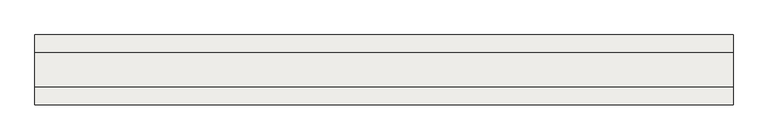
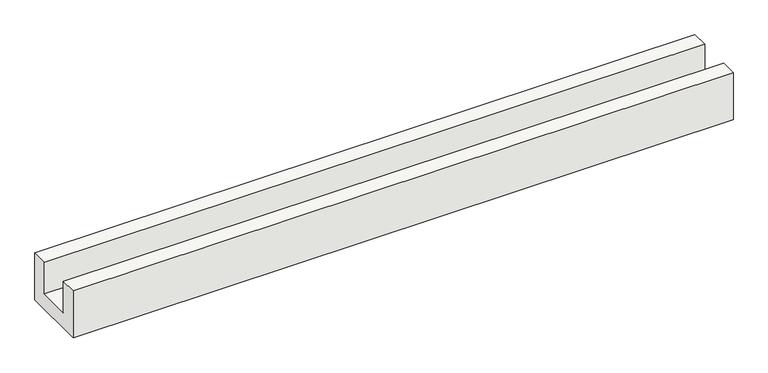
"""IFC4 building model written with IfcOpenShell, lengths in millimetres: slab geometry, 구조 기초 2 : 구조 기초 2."""

from ifc_helpers import new_model, si_unit, frame, origin, place, context, project, spatial, polyline, outline, extrude, source, transform, mapped, element, save


def slab_4cb18c4a(model_context):
    return source(origin(), model_context, "Body", "SweptSolid", [
        extrude(outline(polyline([(8497.8797696, 599.9720055), (8747.8797696, 599.9720055), (8747.8797696, 99.9720055), (9247.8797696, 99.9720055), (9247.8797696, 599.9720055), (9497.8797696, 599.9720055), (9497.8797696, -150.0279945), (8497.8797696, -150.0279945), (8497.8797696, 599.9720055)])), frame((-7005.2480259, 0.0, 0.0), z_axis=(1.0, 0.0, 0.0), x_axis=(0.0, 1.0, 0.0)), (0.0, 0.0, 1.0), 10000.0),
    ])


if __name__ == "__main__":
    model = new_model("IFC4")
    model_context = context("Model", 3, world=origin())
    ifc_project = project(units=[si_unit("LENGTHUNIT", "METRE", prefix="MILLI")], contexts=[model_context])
    site = spatial("IfcSite", under=ifc_project)
    building = spatial("IfcBuilding", under=site)
    placement = place(None, origin())
    slab_shape = slab_4cb18c4a(model_context)
    element("IfcSlab", 1, ObjectType="구조 기초 2 : 구조 기초 2", at=placement, inside=building, context=model_context, shape_type="MappedRepresentation", body=[
        mapped(slab_shape, transform((0.0, 0.0, 0.0), x_axis=(1.0, 0.0, 0.0), y_axis=(0.0, 1.0, 0.0), z_axis=(0.0, 0.0, 1.0))),
    ])
    save(model, "model.ifc")

# Revit data of these elements
# Type "구조 기초 2 : 구조 기초 2"
#   Volume [instance default] = 5.0000 m
#   TWidth [instance default] = 1.0000 m
#   TLength [instance default] = 10.0000 m
#   THeight [instance default] = 0.7500 m
#   DWidth [instance default] = 0.5000 m
#   DHeight [instance default] = 0.5000 m
